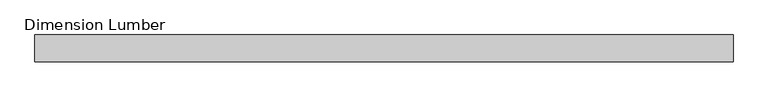
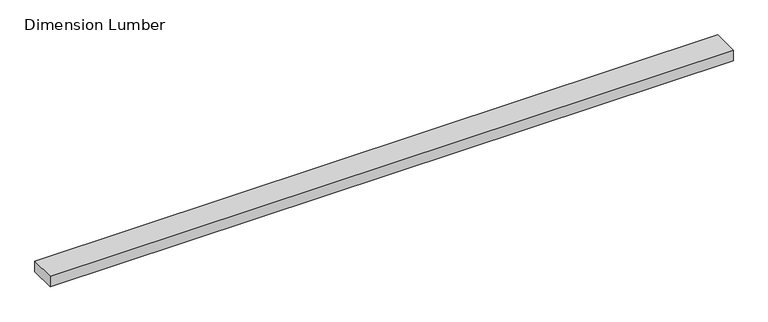
"""IFC4 building model written with IfcOpenShell, lengths in millimetres: beam geometry, Dimension Lumber : Top Supporting Lumbers."""

from ifc_helpers import new_model, si_unit, frame, origin, place, context, project, spatial, polyline, outline, extrude, source, transform, mapped, element, save


def dimension_lumber_3e8a9e7d(model_context):
    return source(origin(), model_context, "Body", "SweptSolid", [
        extrude(outline(polyline([(1158.8750006, 44.45), (1158.8750006, -44.45), (-1139.825, -44.45), (-1139.825, 44.45), (1158.8750006, 44.45)])), frame((0.0, 0.0, -19.05), z_axis=(0.0, 0.0, 1.0), x_axis=(1.0, 0.0, 0.0)), (0.0, 0.0, 1.0), 38.1),
    ])


if __name__ == "__main__":
    model = new_model("IFC4")
    model_context = context("Model", 3, world=origin())
    ifc_project = project(units=[si_unit("LENGTHUNIT", "METRE", prefix="MILLI")], contexts=[model_context])
    site = spatial("IfcSite", under=ifc_project)
    building = spatial("IfcBuilding", under=site)
    placement = place(None, origin())
    dimension_lumber_shape = dimension_lumber_3e8a9e7d(model_context)
    element("IfcBeam", 1, ObjectType="Dimension Lumber : Top Supporting Lumbers", at=placement, inside=building, context=model_context, shape_type="MappedRepresentation", body=[
        mapped(dimension_lumber_shape, transform((0.0, 0.0, 0.0), x_axis=(1.0, 0.0, 0.0), y_axis=(0.0, 1.0, 0.0), z_axis=(0.0, 0.0, 1.0))),
    ])
    save(model, "model.ifc")

# Revit data of these elements
# Type "Dimension Lumber : Top Supporting Lumbers"
#   Assembly Code = "B10"
#   A = 0.0364583 SF
#   Length [instance default] = 5' - 0"
#   b = 0' - 3 1/2"
#   d = 0' - 1 1/2"
#   Structural Material [instance default] = Softwood, Lumber
# Element 1 (IfcBeam, "Dimension Lumber : Top Supporting Lumbers")
#   Structural Material = Douglas Fir #2
#   Materials on its faces: "Douglas Fir #2"
# Materials
#   "Softwood, Lumber": class "Wood", colour RGB 223 192 134, transparency 0, Description = "Pinus Echinata", Cost = 0
#   "Douglas Fir #2": class "Wood", colour RGB 223 192 134, transparency 0, Description = "Pinus Echinata", Cost = 0
